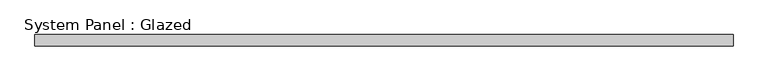
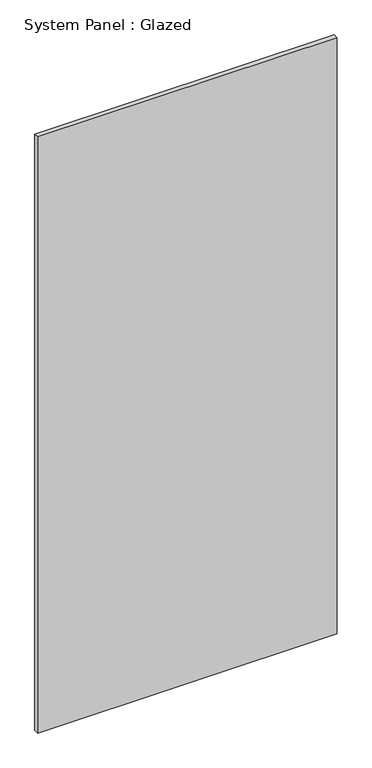
"""IFC4 building model written with IfcOpenShell, lengths in millimetres: plate geometry, System Panel : Glazed."""

from ifc_helpers import new_model, si_unit, origin, origin_with_axes, place, context, project, spatial, polyline, outline, extrude, source, transform, mapped, element, save


def system_panel_glazed_3dc34c55(model_context):
    return source(origin(), model_context, "Body", "SweptSolid", [
        extrude(outline(polyline([(796.9250048, 19.05), (-796.9250048, 19.05), (-796.9250048, 44.45), (796.9250048, 44.45), (796.9250048, 19.05)])), origin_with_axes(), (0.0, 0.0, 1.0), 3352.8),
    ])


if __name__ == "__main__":
    model = new_model("IFC4")
    model_context = context("Model", 3, world=origin())
    ifc_project = project(units=[si_unit("LENGTHUNIT", "METRE", prefix="MILLI")], contexts=[model_context])
    site = spatial("IfcSite", under=ifc_project)
    building = spatial("IfcBuilding", under=site)
    placement = place(None, origin())
    system_panel_glazed_shape = system_panel_glazed_3dc34c55(model_context)
    element("IfcPlate", 1, ObjectType="System Panel : Glazed", at=placement, inside=building, context=model_context, shape_type="MappedRepresentation", body=[
        mapped(system_panel_glazed_shape, transform((0.0, 0.0, 0.0), x_axis=(1.0, 0.0, 0.0), y_axis=(0.0, 1.0, 0.0), z_axis=(0.0, 0.0, 1.0))),
    ])
    save(model, "model.ifc")

# Revit data of these elements
# Type "System Panel : Glazed"
#   Construction Type Id = "GSP4R"
#   Analytic Construction = "1/8 in Pilkington single glazing"
#   Visual Light Transmittance = 0.9
#   Solar Heat Gain Coefficient = 0.86
#   Heat Transfer Coefficient (U) = 1.18115 BTU/(h·ft²·°F)
#   Define Thermal Properties by = 1
# Element 1 (IfcPlate, "System Panel : Glazed")
#   Materials on its faces: "Glass"
# Materials
#   "Glass": class "Glass", colour RGB 0 128 192, transparency 0.75, Description = "Soda Lime Glass", Cost = 0
